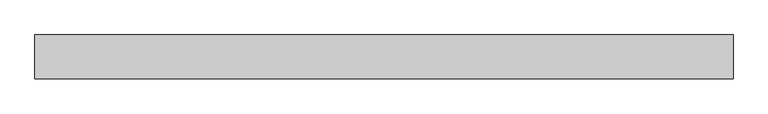
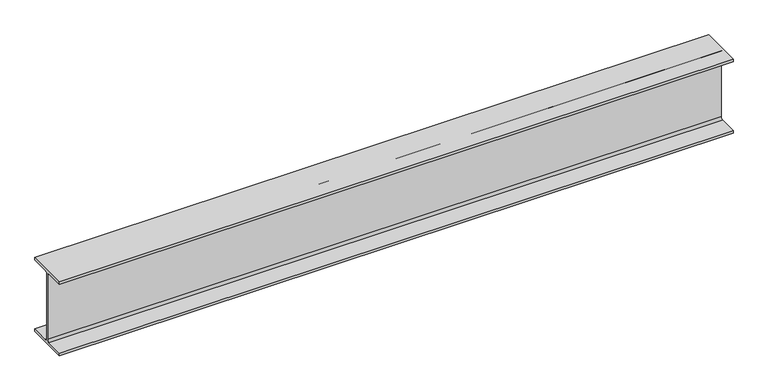
"""IFC4 building model written with IfcOpenShell, lengths in millimetres: beam geometry, Steel Beam_H-KSD3502 : H_SB_ASB_H-194x150x6x9."""

import ifcopenshell
import ifcopenshell.guid

model = None  # the IFC model being written
_history = None  # IfcOwnerHistory: only IFC2X3 demands one
_inside = {}  # id of a spatial element -> (the spatial element, [elements in it])
_under = {}  # id of a project, library or spatial element -> (it, [spatial elements below it])
_declared = {}  # id of a project -> (the project, [libraries it declares])
_typed = {}  # id of a type object -> (the type object, [elements of that type])
_made_of = {}  # id of a material, layer set ... -> (it, [elements and type objects made of it])


def new_model(schema):
    """Start an empty IFC model of exactly this schema.

    Asked for "IFC4X3", IfcOpenShell would pick the latest addendum, in which some entities
    have other attributes; the version numbers below select the first issue.
    IFC2X3 requires an IfcOwnerHistory on every rooted entity: one is made here for all.
    """
    global model, _history
    if schema == "IFC4X3":
        model = ifcopenshell.file(schema_version=(4, 3, 0, 0))
    else:
        model = ifcopenshell.file(schema=schema)
    _inside.clear()
    _under.clear()
    _declared.clear()
    _typed.clear()
    _made_of.clear()
    _history = None
    if model.schema == "IFC2X3":
        org = make("IfcOrganization", Name="unknown")
        user = make(
            "IfcPersonAndOrganization",
            ThePerson=make("IfcPerson", FamilyName="unknown"),
            TheOrganization=org,
        )
        app = make(
            "IfcApplication",
            ApplicationDeveloper=org,
            Version="unknown",
            ApplicationFullName="unknown",
            ApplicationIdentifier="unknown",
        )
        _history = make(
            "IfcOwnerHistory",
            OwningUser=user,
            OwningApplication=app,
            ChangeAction="ADDED",
            CreationDate=0,
        )
    return model


def make(cls, **values):
    """One entity of the class cls with the attributes given. An attribute that is None is left unset."""
    return model.create_entity(
        cls, **{name: value for name, value in values.items() if value is not None}
    )


def rooted(cls, **values):
    """An entity with a GlobalId (a new one), such as an element, a storey or a relation."""
    return make(cls, GlobalId=ifcopenshell.guid.new(), OwnerHistory=_history, **values)


def si_unit(unit_type, name, prefix=None):
    """IfcSIUnit, for example si_unit("LENGTHUNIT", "METRE", prefix="MILLI")."""
    return make("IfcSIUnit", UnitType=unit_type, Prefix=prefix, Name=name)


def assignment(units):
    """IfcUnitAssignment: the units of a project."""
    return None if units is None else make("IfcUnitAssignment", Units=units)


def point(xyz):
    """IfcCartesianPoint."""
    return None if xyz is None else make("IfcCartesianPoint", Coordinates=xyz)


def direction(xyz):
    """IfcDirection."""
    return None if xyz is None else make("IfcDirection", DirectionRatios=xyz)


def frame(location, z_axis=None, x_axis=None):
    """IfcAxis2Placement3D, a coordinate frame: its origin and axes. An axis left out is left unset."""
    return make(
        "IfcAxis2Placement3D",
        Location=point(location),
        Axis=direction(z_axis),
        RefDirection=direction(x_axis),
    )


def frame_2d(location, x_axis=None):
    """IfcAxis2Placement2D, a coordinate frame in the plane: its origin and x axis."""
    return make(
        "IfcAxis2Placement2D", Location=point(location), RefDirection=direction(x_axis)
    )


def origin():
    """The frame at (0, 0, 0) with its axes left unset."""
    return frame((0.0, 0.0, 0.0))


def place(relative_to, where):
    """IfcLocalPlacement: puts the frame where relative to a parent placement (None: the world)."""
    return make(
        "IfcLocalPlacement", PlacementRelTo=relative_to, RelativePlacement=where
    )


def context(
    kind, dimensions, precision=None, world=None, true_north=None, identifier=None
):
    """IfcGeometricRepresentationContext, for example the 3D "Model" context."""
    return make(
        "IfcGeometricRepresentationContext",
        ContextIdentifier=identifier,
        ContextType=kind,
        CoordinateSpaceDimension=dimensions,
        Precision=precision,
        WorldCoordinateSystem=world,
        TrueNorth=true_north,
    )


def project(units=None, contexts=None):
    """IfcProject with its units and contexts."""
    return rooted(
        "IfcProject",
        Name="project",
        RepresentationContexts=contexts,
        UnitsInContext=assignment(units),
    )


def spatial(cls, under=None, at=None, **own):
    """A site, building, storey or space (cls), placed at a placement, below another one or the project."""
    s = rooted(cls, ObjectPlacement=at, **own)
    if under is not None:
        _under.setdefault(under.id(), (under, []))[1].append(s)
    return s


def polyline(points):
    """IfcPolyline through the points."""
    return make("IfcPolyline", Points=[point(p) for p in points])


def circle_curve(where, radius):
    """IfcCircle in the frame where."""
    return make("IfcCircle", Position=where, Radius=radius)


def trimmed(basis, trim1, trim2, sense, master):
    """IfcTrimmedCurve: the piece of a basis curve between two trims."""
    return make(
        "IfcTrimmedCurve",
        BasisCurve=basis,
        Trim1=trim1,
        Trim2=trim2,
        SenseAgreement=sense,
        MasterRepresentation=master,
    )


def segment(curve, same_sense, transition):
    """IfcCompositeCurveSegment."""
    return make(
        "IfcCompositeCurveSegment",
        Transition=transition,
        SameSense=same_sense,
        ParentCurve=curve,
    )


def composite_curve(segments, self_intersect=None):
    """IfcCompositeCurve: segments joined end to end."""
    return make("IfcCompositeCurve", Segments=segments, SelfIntersect=self_intersect)


def outline(outer, holes=None, kind="AREA"):
    """IfcArbitraryClosedProfileDef: a profile drawn as a closed curve; with holes, ...WithVoids."""
    if holes is None:
        return make("IfcArbitraryClosedProfileDef", ProfileType=kind, OuterCurve=outer)
    return make(
        "IfcArbitraryProfileDefWithVoids",
        ProfileType=kind,
        OuterCurve=outer,
        InnerCurves=holes,
    )


def extrude(swept, where, along, depth):
    """IfcExtrudedAreaSolid: the profile swept, set in the frame where, extruded along a direction by depth."""
    return make(
        "IfcExtrudedAreaSolid",
        SweptArea=swept,
        Position=where,
        ExtrudedDirection=direction(along),
        Depth=depth,
    )


def shape(context_of_items, identifier, shape_type, items):
    """IfcShapeRepresentation: the items that make up one representation, for example the "Body"."""
    return make(
        "IfcShapeRepresentation",
        ContextOfItems=context_of_items,
        RepresentationIdentifier=identifier,
        RepresentationType=shape_type,
        Items=items,
    )


def source(mapping_origin, context_of_items, identifier, shape_type, items):
    """IfcRepresentationMap: a shape defined once, which mapped items show again and again."""
    return make(
        "IfcRepresentationMap",
        MappingOrigin=mapping_origin,
        MappedRepresentation=shape(context_of_items, identifier, shape_type, items),
    )


def transform(
    local_origin,
    x_axis=None,
    y_axis=None,
    z_axis=None,
    scale=None,
    scale2=None,
    scale3=None,
    uniform=True,
):
    """IfcCartesianTransformationOperator3D, or its non-uniform kind. x_axis, y_axis, z_axis: its Axis1, 2, 3."""
    if uniform:
        return make(
            "IfcCartesianTransformationOperator3D",
            Axis1=direction(x_axis),
            Axis2=direction(y_axis),
            LocalOrigin=point(local_origin),
            Scale=scale,
            Axis3=direction(z_axis),
        )
    return make(
        "IfcCartesianTransformationOperator3DnonUniform",
        Axis1=direction(x_axis),
        Axis2=direction(y_axis),
        LocalOrigin=point(local_origin),
        Scale=scale,
        Axis3=direction(z_axis),
        Scale2=scale2,
        Scale3=scale3,
    )


def mapped(mapping_source, mapping_target):
    """IfcMappedItem: shows the shape of a source again, moved by a transform."""
    return make(
        "IfcMappedItem", MappingSource=mapping_source, MappingTarget=mapping_target
    )


def made_of(thing, what):
    """Note that an element or type object is made of a material, layer set ...; save() writes the relation."""
    if what is not None:
        _made_of.setdefault(what.id(), (what, []))[1].append(thing)
    return thing


def element(
    cls,
    number,
    at=None,
    inside=None,
    cuts=None,
    type_object=None,
    material=None,
    context=None,
    identifier="Body",
    shape_type=None,
    held_by="IfcProductDefinitionShape",
    body=None,
    shapes=None,
    **own,
):
    """One element of the class cls, such as IfcWall. Its Tag is "e" and its number.

    at: its placement. inside: the storey or other place that contains it. cuts: it is an
    opening in that element (IfcRelVoidsElement). A single representation is given by context,
    identifier, shape_type and body (its items); several are given by shapes. held_by: the class
    of the entity that holds the representations. save() writes the other relations.
    """
    e = rooted(cls, Tag="e%d" % number, ObjectPlacement=at, **own)
    if body is not None:
        shapes = [shape(context, identifier, shape_type, body)]
    if shapes is not None:
        e.Representation = make(held_by, Representations=shapes)
    if inside is not None:
        _inside.setdefault(inside.id(), (inside, []))[1].append(e)
    if cuts is not None:
        rooted(
            "IfcRelVoidsElement", RelatingBuildingElement=cuts, RelatedOpeningElement=e
        )
    if type_object is not None:
        _typed.setdefault(type_object.id(), (type_object, []))[1].append(e)
    return made_of(e, material)


def aggregate(whole, parts):
    """IfcRelAggregates: a whole, such as a stair, and the parts it consists of."""
    return rooted("IfcRelAggregates", RelatingObject=whole, RelatedObjects=parts)


def save(model, path):
    """Write the relations noted so far, then the file.

    IfcRelAggregates (storeys below a building ...), IfcRelContainedInSpatialStructure (elements
    in a storey), IfcRelDefinesByType, IfcRelAssociatesMaterial and IfcRelDeclares: one each for
    every whole, place, type object, material and project.
    """
    for whole, parts in _under.values():
        aggregate(whole, parts)
    for where, things in _inside.values():
        rooted(
            "IfcRelContainedInSpatialStructure",
            RelatedElements=things,
            RelatingStructure=where,
        )
    for kind, things in _typed.values():
        rooted("IfcRelDefinesByType", RelatedObjects=things, RelatingType=kind)
    for what, things in _made_of.values():
        rooted("IfcRelAssociatesMaterial", RelatedObjects=things, RelatingMaterial=what)
    for by, libraries in _declared.values():
        rooted("IfcRelDeclares", RelatingContext=by, RelatedDefinitions=libraries)
    model.write(path)


def beam_f3b47e3d(model_context):
    return source(origin(), model_context, "Body", "SweptSolid", [
        extrude(outline(composite_curve([segment(polyline([(-82.5, -141.5), (-11.9, -141.5)]), True, "CONTINUOUS"), segment(trimmed(circle_curve(frame_2d((-11.9, -132.6)), 8.9), [point((-11.9, -141.5))], [point((-3.0, -132.6))], True, "CARTESIAN"), True, "CONTINUOUS"), segment(polyline([(-3.0, -132.6), (-3.0, 132.6)]), True, "CONTINUOUS"), segment(trimmed(circle_curve(frame_2d((-11.9, 132.6)), 8.9), [point((-3.0, 132.6))], [point((-11.9, 141.5))], True, "CARTESIAN"), True, "CONTINUOUS"), segment(polyline([(-11.9, 141.5), (-82.5, 141.5), (-82.5, 151.7), (82.5, 151.7), (82.5, 141.5), (11.9, 141.5)]), True, "CONTINUOUS"), segment(trimmed(circle_curve(frame_2d((11.9, 132.6)), 8.9), [point((11.9, 141.5))], [point((3.0, 132.6))], True, "CARTESIAN"), True, "CONTINUOUS"), segment(polyline([(3.0, 132.6), (3.0, -132.6)]), True, "CONTINUOUS"), segment(trimmed(circle_curve(frame_2d((11.9, -132.6)), 8.9), [point((3.0, -132.6))], [point((11.9, -141.5))], True, "CARTESIAN"), True, "CONTINUOUS"), segment(polyline([(11.9, -141.5), (82.5, -141.5), (82.5, -151.7), (-82.5, -151.7), (-82.5, -141.5)]), True, "CONTINUOUS")], self_intersect=False)), frame((-1068.0314701, 0.0, 0.0), z_axis=(1.0, 0.0, 0.0), x_axis=(0.0, 1.0, 0.0)), (0.0, 0.0, 1.0), 2617.0588612),
    ])


if __name__ == "__main__":
    model = new_model("IFC4")
    model_context = context("Model", 3, world=origin())
    ifc_project = project(units=[si_unit("LENGTHUNIT", "METRE", prefix="MILLI")], contexts=[model_context])
    site = spatial("IfcSite", under=ifc_project)
    building = spatial("IfcBuilding", under=site)
    placement = place(None, origin())
    beam_shape = beam_f3b47e3d(model_context)
    element("IfcBeam", 1, ObjectType="Steel Beam_H-KSD3502 : H_SB_ASB_H-194x150x6x9", at=placement, inside=building, context=model_context, shape_type="MappedRepresentation", body=[
        mapped(beam_shape, transform((0.0, 0.0, 0.0), x_axis=(1.0, 0.0, 0.0), y_axis=(0.0, 1.0, 0.0), z_axis=(0.0, 0.0, 1.0))),
    ])
    save(model, "model.ifc")

# Revit data of these elements
# Type "Steel Beam_H-KSD3502 : H_SB_ASB_H-194x150x6x9"
#   Width = 15.0 cm
#   Web Thickness = 0.6 cm
#   Web Fillet = 1.3 cm
#   Warping Constant = 43316.0 cm⁶
#   Torsional Moment of Inertia = 8.622 cm⁴
#   Torsional Modulus = 1.0 cm³
#   Section Area = 39.01 cm²
#   Plastic Modulus weak axis = 104.0 cm³
#   Plastic Modulus strong axis = 309.0 cm³
#   Perimeter = 0.95 m²/m
#   Nominal Weight = 30.60 kgf/m
#   Moment of Inertia weak axis = 507.00 cm⁴
#   Moment of Inertia strong axis = 2690.00 cm⁴
#   Height = 19.4 cm
#   Flange Thickness = 0.9 cm
#   Elastic Modulus weak axis = 67.6 cm³
#   Elastic Modulus strong axis = 277.0 cm³
#   Centroid Vertical = 9.7 cm
#   Centroid Horizontal = 7.5 cm
#   Length [instance default] = 1.5240 m
#   Structural Material [instance default] = Steel, 45-345
#   Assembly Code = ""
# Element 1 (IfcBeam, "Steel Beam_H-KSD3502 : H_SB_ASB_H-194x150x6x9")
#   Structural Material = none
# Materials
#   "Steel, 45-345": class "Metal", colour RGB 189 187 185, transparency 0, Description = "Steel 345 MPa", Cost = 0
